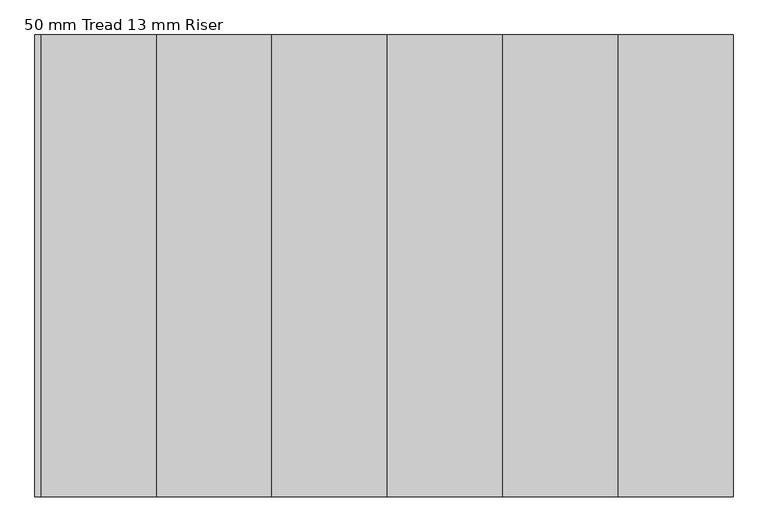
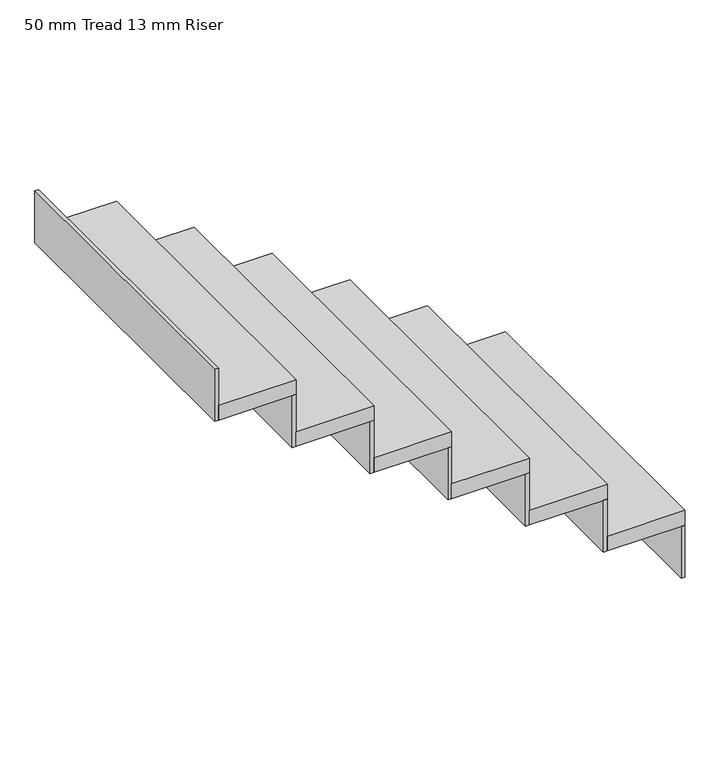
"""IFC4 building model written with IfcOpenShell, lengths in millimetres: stair flight geometry, 50 mm Tread 13 mm Riser."""

import ifcopenshell
import ifcopenshell.guid

model = None  # the IFC model being written
_history = None  # IfcOwnerHistory: only IFC2X3 demands one
_inside = {}  # id of a spatial element -> (the spatial element, [elements in it])
_under = {}  # id of a project, library or spatial element -> (it, [spatial elements below it])
_declared = {}  # id of a project -> (the project, [libraries it declares])
_typed = {}  # id of a type object -> (the type object, [elements of that type])
_made_of = {}  # id of a material, layer set ... -> (it, [elements and type objects made of it])


def new_model(schema):
    """Start an empty IFC model of exactly this schema.

    Asked for "IFC4X3", IfcOpenShell would pick the latest addendum, in which some entities
    have other attributes; the version numbers below select the first issue.
    IFC2X3 requires an IfcOwnerHistory on every rooted entity: one is made here for all.
    """
    global model, _history
    if schema == "IFC4X3":
        model = ifcopenshell.file(schema_version=(4, 3, 0, 0))
    else:
        model = ifcopenshell.file(schema=schema)
    _inside.clear()
    _under.clear()
    _declared.clear()
    _typed.clear()
    _made_of.clear()
    _history = None
    if model.schema == "IFC2X3":
        org = make("IfcOrganization", Name="unknown")
        user = make(
            "IfcPersonAndOrganization",
            ThePerson=make("IfcPerson", FamilyName="unknown"),
            TheOrganization=org,
        )
        app = make(
            "IfcApplication",
            ApplicationDeveloper=org,
            Version="unknown",
            ApplicationFullName="unknown",
            ApplicationIdentifier="unknown",
        )
        _history = make(
            "IfcOwnerHistory",
            OwningUser=user,
            OwningApplication=app,
            ChangeAction="ADDED",
            CreationDate=0,
        )
    return model


def make(cls, **values):
    """One entity of the class cls with the attributes given. An attribute that is None is left unset."""
    return model.create_entity(
        cls, **{name: value for name, value in values.items() if value is not None}
    )


def rooted(cls, **values):
    """An entity with a GlobalId (a new one), such as an element, a storey or a relation."""
    return make(cls, GlobalId=ifcopenshell.guid.new(), OwnerHistory=_history, **values)


def si_unit(unit_type, name, prefix=None):
    """IfcSIUnit, for example si_unit("LENGTHUNIT", "METRE", prefix="MILLI")."""
    return make("IfcSIUnit", UnitType=unit_type, Prefix=prefix, Name=name)


def assignment(units):
    """IfcUnitAssignment: the units of a project."""
    return None if units is None else make("IfcUnitAssignment", Units=units)


def point(xyz):
    """IfcCartesianPoint."""
    return None if xyz is None else make("IfcCartesianPoint", Coordinates=xyz)


def direction(xyz):
    """IfcDirection."""
    return None if xyz is None else make("IfcDirection", DirectionRatios=xyz)


def frame(location, z_axis=None, x_axis=None):
    """IfcAxis2Placement3D, a coordinate frame: its origin and axes. An axis left out is left unset."""
    return make(
        "IfcAxis2Placement3D",
        Location=point(location),
        Axis=direction(z_axis),
        RefDirection=direction(x_axis),
    )


def origin():
    """The frame at (0, 0, 0) with its axes left unset."""
    return frame((0.0, 0.0, 0.0))


def place(relative_to, where):
    """IfcLocalPlacement: puts the frame where relative to a parent placement (None: the world)."""
    return make(
        "IfcLocalPlacement", PlacementRelTo=relative_to, RelativePlacement=where
    )


def context(
    kind, dimensions, precision=None, world=None, true_north=None, identifier=None
):
    """IfcGeometricRepresentationContext, for example the 3D "Model" context."""
    return make(
        "IfcGeometricRepresentationContext",
        ContextIdentifier=identifier,
        ContextType=kind,
        CoordinateSpaceDimension=dimensions,
        Precision=precision,
        WorldCoordinateSystem=world,
        TrueNorth=true_north,
    )


def project(units=None, contexts=None):
    """IfcProject with its units and contexts."""
    return rooted(
        "IfcProject",
        Name="project",
        RepresentationContexts=contexts,
        UnitsInContext=assignment(units),
    )


def spatial(cls, under=None, at=None, **own):
    """A site, building, storey or space (cls), placed at a placement, below another one or the project."""
    s = rooted(cls, ObjectPlacement=at, **own)
    if under is not None:
        _under.setdefault(under.id(), (under, []))[1].append(s)
    return s


def polyline(points):
    """IfcPolyline through the points."""
    return make("IfcPolyline", Points=[point(p) for p in points])


def outline(outer, holes=None, kind="AREA"):
    """IfcArbitraryClosedProfileDef: a profile drawn as a closed curve; with holes, ...WithVoids."""
    if holes is None:
        return make("IfcArbitraryClosedProfileDef", ProfileType=kind, OuterCurve=outer)
    return make(
        "IfcArbitraryProfileDefWithVoids",
        ProfileType=kind,
        OuterCurve=outer,
        InnerCurves=holes,
    )


def extrude(swept, where, along, depth):
    """IfcExtrudedAreaSolid: the profile swept, set in the frame where, extruded along a direction by depth."""
    return make(
        "IfcExtrudedAreaSolid",
        SweptArea=swept,
        Position=where,
        ExtrudedDirection=direction(along),
        Depth=depth,
    )


def shape(context_of_items, identifier, shape_type, items):
    """IfcShapeRepresentation: the items that make up one representation, for example the "Body"."""
    return make(
        "IfcShapeRepresentation",
        ContextOfItems=context_of_items,
        RepresentationIdentifier=identifier,
        RepresentationType=shape_type,
        Items=items,
    )


def source(mapping_origin, context_of_items, identifier, shape_type, items):
    """IfcRepresentationMap: a shape defined once, which mapped items show again and again."""
    return make(
        "IfcRepresentationMap",
        MappingOrigin=mapping_origin,
        MappedRepresentation=shape(context_of_items, identifier, shape_type, items),
    )


def transform(
    local_origin,
    x_axis=None,
    y_axis=None,
    z_axis=None,
    scale=None,
    scale2=None,
    scale3=None,
    uniform=True,
):
    """IfcCartesianTransformationOperator3D, or its non-uniform kind. x_axis, y_axis, z_axis: its Axis1, 2, 3."""
    if uniform:
        return make(
            "IfcCartesianTransformationOperator3D",
            Axis1=direction(x_axis),
            Axis2=direction(y_axis),
            LocalOrigin=point(local_origin),
            Scale=scale,
            Axis3=direction(z_axis),
        )
    return make(
        "IfcCartesianTransformationOperator3DnonUniform",
        Axis1=direction(x_axis),
        Axis2=direction(y_axis),
        LocalOrigin=point(local_origin),
        Scale=scale,
        Axis3=direction(z_axis),
        Scale2=scale2,
        Scale3=scale3,
    )


def mapped(mapping_source, mapping_target):
    """IfcMappedItem: shows the shape of a source again, moved by a transform."""
    return make(
        "IfcMappedItem", MappingSource=mapping_source, MappingTarget=mapping_target
    )


def made_of(thing, what):
    """Note that an element or type object is made of a material, layer set ...; save() writes the relation."""
    if what is not None:
        _made_of.setdefault(what.id(), (what, []))[1].append(thing)
    return thing


def element(
    cls,
    number,
    at=None,
    inside=None,
    cuts=None,
    type_object=None,
    material=None,
    context=None,
    identifier="Body",
    shape_type=None,
    held_by="IfcProductDefinitionShape",
    body=None,
    shapes=None,
    **own,
):
    """One element of the class cls, such as IfcWall. Its Tag is "e" and its number.

    at: its placement. inside: the storey or other place that contains it. cuts: it is an
    opening in that element (IfcRelVoidsElement). A single representation is given by context,
    identifier, shape_type and body (its items); several are given by shapes. held_by: the class
    of the entity that holds the representations. save() writes the other relations.
    """
    e = rooted(cls, Tag="e%d" % number, ObjectPlacement=at, **own)
    if body is not None:
        shapes = [shape(context, identifier, shape_type, body)]
    if shapes is not None:
        e.Representation = make(held_by, Representations=shapes)
    if inside is not None:
        _inside.setdefault(inside.id(), (inside, []))[1].append(e)
    if cuts is not None:
        rooted(
            "IfcRelVoidsElement", RelatingBuildingElement=cuts, RelatedOpeningElement=e
        )
    if type_object is not None:
        _typed.setdefault(type_object.id(), (type_object, []))[1].append(e)
    return made_of(e, material)


def aggregate(whole, parts):
    """IfcRelAggregates: a whole, such as a stair, and the parts it consists of."""
    return rooted("IfcRelAggregates", RelatingObject=whole, RelatedObjects=parts)


def save(model, path):
    """Write the relations noted so far, then the file.

    IfcRelAggregates (storeys below a building ...), IfcRelContainedInSpatialStructure (elements
    in a storey), IfcRelDefinesByType, IfcRelAssociatesMaterial and IfcRelDeclares: one each for
    every whole, place, type object, material and project.
    """
    for whole, parts in _under.values():
        aggregate(whole, parts)
    for where, things in _inside.values():
        rooted(
            "IfcRelContainedInSpatialStructure",
            RelatedElements=things,
            RelatingStructure=where,
        )
    for kind, things in _typed.values():
        rooted("IfcRelDefinesByType", RelatedObjects=things, RelatingType=kind)
    for what, things in _made_of.values():
        rooted("IfcRelAssociatesMaterial", RelatedObjects=things, RelatingMaterial=what)
    for by, libraries in _declared.values():
        rooted("IfcRelDeclares", RelatingContext=by, RelatedDefinitions=libraries)
    model.write(path)


def stair_flight_50_mm_tread_13_mm_riser_d2236daa(model_context):
    return source(origin(), model_context, "Body", "SweptSolid", [
        extrude(outline(polyline([(30681.6667192, -1501.242277), (30694.1667192, -1501.242277), (30694.1667192, -2501.242277), (30681.6667192, -2501.242277), (30681.6667192, -1501.242277)])), frame((0.0, 0.0, 1714.7058824), z_axis=(0.0, 0.0, 1.0), x_axis=(1.0, 0.0, 0.0)), (0.0, 0.0, 1.0), 176.4705882),
        extrude(outline(polyline([(30444.1667192, -2501.242277), (30444.1667192, -1501.242277), (30694.1667192, -1501.242277), (30694.1667192, -2501.242277), (30444.1667192, -2501.242277)])), frame((0.0, 0.0, 1891.1764706), z_axis=(0.0, 0.0, 1.0), x_axis=(1.0, 0.0, 0.0)), (0.0, 0.0, 1.0), 50.0),
        extrude(outline(polyline([(30431.6667192, -1501.242277), (30444.1667192, -1501.242277), (30444.1667192, -2501.242277), (30431.6667192, -2501.242277), (30431.6667192, -1501.242277)])), frame((0.0, 0.0, 1891.1764706), z_axis=(0.0, 0.0, 1.0), x_axis=(1.0, 0.0, 0.0)), (0.0, 0.0, 1.0), 176.4705882),
        extrude(outline(polyline([(30194.1667192, -2501.242277), (30194.1667192, -1501.242277), (30444.1667192, -1501.242277), (30444.1667192, -2501.242277), (30194.1667192, -2501.242277)])), frame((0.0, 0.0, 2067.6470588), z_axis=(0.0, 0.0, 1.0), x_axis=(1.0, 0.0, 0.0)), (0.0, 0.0, 1.0), 50.0),
        extrude(outline(polyline([(30181.6667192, -1501.242277), (30194.1667192, -1501.242277), (30194.1667192, -2501.242277), (30181.6667192, -2501.242277), (30181.6667192, -1501.242277)])), frame((0.0, 0.0, 2067.6470588), z_axis=(0.0, 0.0, 1.0), x_axis=(1.0, 0.0, 0.0)), (0.0, 0.0, 1.0), 176.4705882),
        extrude(outline(polyline([(29944.1667192, -2501.242277), (29944.1667192, -1501.242277), (30194.1667192, -1501.242277), (30194.1667192, -2501.242277), (29944.1667192, -2501.242277)])), frame((0.0, 0.0, 2244.1176471), z_axis=(0.0, 0.0, 1.0), x_axis=(1.0, 0.0, 0.0)), (0.0, 0.0, 1.0), 50.0),
        extrude(outline(polyline([(29931.6667192, -1501.242277), (29944.1667192, -1501.242277), (29944.1667192, -2501.242277), (29931.6667192, -2501.242277), (29931.6667192, -1501.242277)])), frame((0.0, 0.0, 2244.1176471), z_axis=(0.0, 0.0, 1.0), x_axis=(1.0, 0.0, 0.0)), (0.0, 0.0, 1.0), 176.4705882),
        extrude(outline(polyline([(29694.1667192, -2501.242277), (29694.1667192, -1501.242277), (29944.1667192, -1501.242277), (29944.1667192, -2501.242277), (29694.1667192, -2501.242277)])), frame((0.0, 0.0, 2420.5882353), z_axis=(0.0, 0.0, 1.0), x_axis=(1.0, 0.0, 0.0)), (0.0, 0.0, 1.0), 50.0),
        extrude(outline(polyline([(29681.6667192, -1501.242277), (29694.1667192, -1501.242277), (29694.1667192, -2501.242277), (29681.6667192, -2501.242277), (29681.6667192, -1501.242277)])), frame((0.0, 0.0, 2420.5882353), z_axis=(0.0, 0.0, 1.0), x_axis=(1.0, 0.0, 0.0)), (0.0, 0.0, 1.0), 176.4705882),
        extrude(outline(polyline([(29444.1667192, -2501.242277), (29444.1667192, -1501.242277), (29694.1667192, -1501.242277), (29694.1667192, -2501.242277), (29444.1667192, -2501.242277)])), frame((0.0, 0.0, 2597.0588235), z_axis=(0.0, 0.0, 1.0), x_axis=(1.0, 0.0, 0.0)), (0.0, 0.0, 1.0), 50.0),
        extrude(outline(polyline([(29431.6667192, -1501.242277), (29444.1667192, -1501.242277), (29444.1667192, -2501.242277), (29431.6667192, -2501.242277), (29431.6667192, -1501.242277)])), frame((0.0, 0.0, 2597.0588235), z_axis=(0.0, 0.0, 1.0), x_axis=(1.0, 0.0, 0.0)), (0.0, 0.0, 1.0), 176.4705882),
        extrude(outline(polyline([(29181.6667192, -1501.242277), (29194.1667192, -1501.242277), (29194.1667192, -2501.242277), (29181.6667192, -2501.242277), (29181.6667192, -1501.242277)])), frame((0.0, 0.0, 2773.5294118), z_axis=(0.0, 0.0, 1.0), x_axis=(1.0, 0.0, 0.0)), (0.0, 0.0, 1.0), 176.4705882),
        extrude(outline(polyline([(29194.1667192, -2501.242277), (29194.1667192, -1501.242277), (29444.1667192, -1501.242277), (29444.1667192, -2501.242277), (29194.1667192, -2501.242277)])), frame((0.0, 0.0, 2773.5294118), z_axis=(0.0, 0.0, 1.0), x_axis=(1.0, 0.0, 0.0)), (0.0, 0.0, 1.0), 50.0),
    ])


if __name__ == "__main__":
    model = new_model("IFC4")
    model_context = context("Model", 3, world=origin())
    ifc_project = project(units=[si_unit("LENGTHUNIT", "METRE", prefix="MILLI")], contexts=[model_context])
    site = spatial("IfcSite", under=ifc_project)
    building = spatial("IfcBuilding", under=site)
    placement = place(None, origin())
    stair_flight_50_mm_tread_13_mm_riser_shape = stair_flight_50_mm_tread_13_mm_riser_d2236daa(model_context)
    element("IfcStairFlight", 1, ObjectType="50 mm Tread 13 mm Riser", at=placement, inside=building, context=model_context, shape_type="MappedRepresentation", body=[
        mapped(stair_flight_50_mm_tread_13_mm_riser_shape, transform((0.0, 0.0, 0.0), x_axis=(1.0, 0.0, 0.0), y_axis=(0.0, 1.0, 0.0), z_axis=(0.0, 0.0, 1.0))),
    ])
    save(model, "model.ifc")
